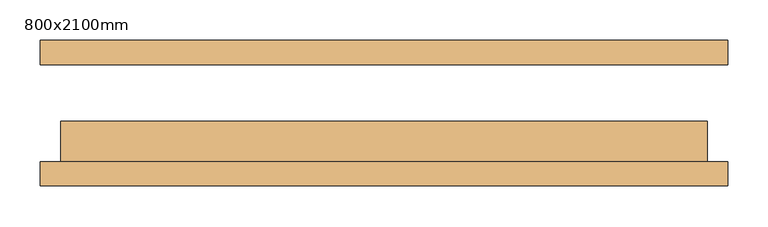
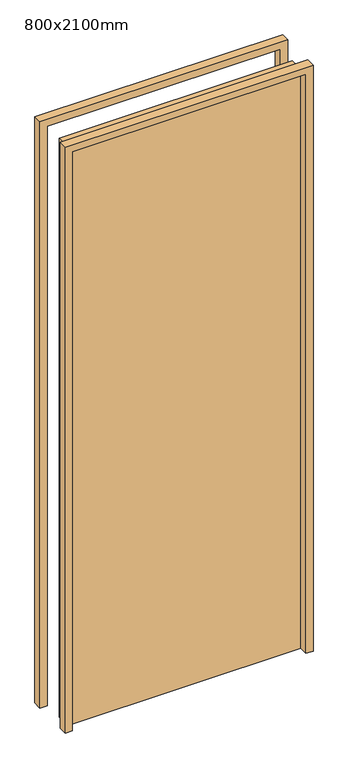
"""IFC4 building model written with IfcOpenShell, lengths in millimetres: door geometry, WWm-SingleSolid-Flush : 800x2100mm."""

from ifc_helpers import new_model, si_unit, frame, origin, origin_with_axes, place, context, project, spatial, polyline, outline, extrude, source, transform, mapped, element, save


def door_800x2100mm_ee10ec43(model_context):
    return source(origin(), model_context, "Body", "SweptSolid", [
        extrude(outline(polyline([(2125.0, -425.0), (0.0, -425.0), (0.0, -400.0), (2100.0, -400.0), (2100.0, 400.0), (0.0, 400.0), (0.0, 425.0), (2125.0, 425.0), (2125.0, -425.0)])), frame((0.0, -90.0, 0.0), z_axis=(0.0, 1.0, 0.0), x_axis=(0.0, 0.0, 1.0)), (0.0, 0.0, 1.0), 30.0),
        extrude(outline(polyline([(2125.0, 425.0), (2125.0, -425.0), (0.0, -425.0), (0.0, -400.0), (2100.0, -400.0), (2100.0, 400.0), (0.0, 400.0), (0.0, 425.0), (2125.0, 425.0)])), frame((0.0, 60.0, 0.0), z_axis=(0.0, 1.0, 0.0), x_axis=(0.0, 0.0, 1.0)), (0.0, 0.0, 1.0), 30.0),
        extrude(outline(polyline([(400.0, -10.0), (400.0, -60.0), (-400.0, -60.0), (-400.0, -10.0), (400.0, -10.0)])), origin_with_axes(), (0.0, 0.0, 1.0), 2100.0),
    ])


if __name__ == "__main__":
    model = new_model("IFC4")
    model_context = context("Model", 3, world=origin())
    ifc_project = project(units=[si_unit("LENGTHUNIT", "METRE", prefix="MILLI")], contexts=[model_context])
    site = spatial("IfcSite", under=ifc_project)
    building = spatial("IfcBuilding", under=site)
    placement = place(None, origin())
    door_800x2100mm_shape = door_800x2100mm_ee10ec43(model_context)
    element("IfcDoor", 1, ObjectType="WWm-SingleSolid-Flush : 800x2100mm", at=placement, inside=building, context=model_context, shape_type="MappedRepresentation", body=[
        mapped(door_800x2100mm_shape, transform((0.0, 0.0, 0.0), x_axis=(1.0, 0.0, 0.0), y_axis=(0.0, 1.0, 0.0), z_axis=(0.0, 0.0, 1.0))),
    ])
    save(model, "model.ifc")

# Revit data of these elements
# Type "WWm-SingleSolid-Flush : 800x2100mm"
#   Type Mark = "EX1-54"
#   Construction Type Id = "MDOOR"
#   Assembly Code = "C1020"
#   Analytic Construction = "Metal"
#   Thickness = 50 mm
#   Thermal Resistance (R) = 0.270117 (m²·K)/W
#   Heat Transfer Coefficient (U) = 3.7021 W/(m²·K)
#   Height = 2100 mm
#   Trim Projection Ext = 30 mm
#   Trim Projection Int = 30 mm
#   Trim Width = 25 mm
#   Width = 800 mm
#   Not 90 Degree [instance default] = no
#   90 Degree [instance default] = yes
#   Door Material = WW-EC-RGB-White
#   Frame Material = WW-EC-RGB-White
#   Visual Light Transmittance = 0
#   Solar Heat Gain Coefficient = 0
#   Function = (empty or 0)
#   Wall Closure = (empty or 0)
# Element 1 (IfcDoor, "WWm-SingleSolid-Flush : 800x2100mm")
#   Materials on its faces: "WW-EC-RGB-White"
# Materials
#   "WW-EC-RGB-White": class "Generic", colour RGB 255 255 255, transparency 0, Comments = "If region requests off-white, swith asset color to RGB 231-228-220", Description = "Generic Color", Cost = 0
